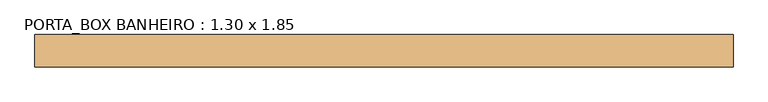
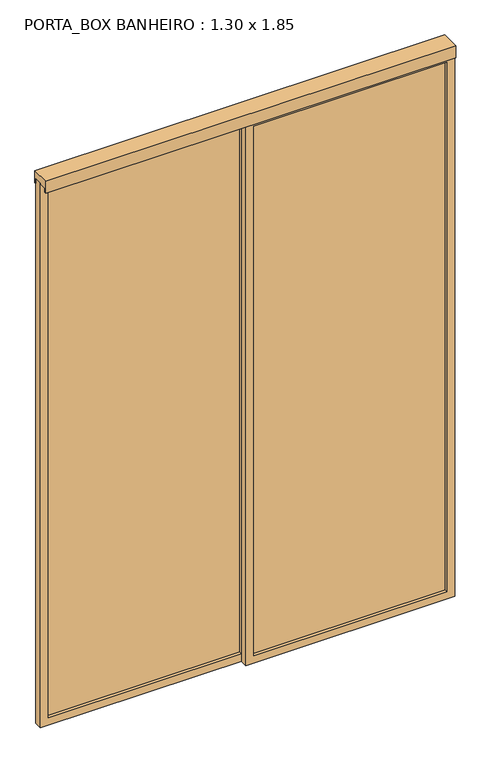
"""IFC4 building model written with IfcOpenShell, lengths in millimetres: door geometry, PORTA_BOX BANHEIRO : 1.30 x 1.85."""

import ifcopenshell
import ifcopenshell.guid

model = None  # the IFC model being written
_history = None  # IfcOwnerHistory: only IFC2X3 demands one
_inside = {}  # id of a spatial element -> (the spatial element, [elements in it])
_under = {}  # id of a project, library or spatial element -> (it, [spatial elements below it])
_declared = {}  # id of a project -> (the project, [libraries it declares])
_typed = {}  # id of a type object -> (the type object, [elements of that type])
_made_of = {}  # id of a material, layer set ... -> (it, [elements and type objects made of it])


def new_model(schema):
    """Start an empty IFC model of exactly this schema.

    Asked for "IFC4X3", IfcOpenShell would pick the latest addendum, in which some entities
    have other attributes; the version numbers below select the first issue.
    IFC2X3 requires an IfcOwnerHistory on every rooted entity: one is made here for all.
    """
    global model, _history
    if schema == "IFC4X3":
        model = ifcopenshell.file(schema_version=(4, 3, 0, 0))
    else:
        model = ifcopenshell.file(schema=schema)
    _inside.clear()
    _under.clear()
    _declared.clear()
    _typed.clear()
    _made_of.clear()
    _history = None
    if model.schema == "IFC2X3":
        org = make("IfcOrganization", Name="unknown")
        user = make(
            "IfcPersonAndOrganization",
            ThePerson=make("IfcPerson", FamilyName="unknown"),
            TheOrganization=org,
        )
        app = make(
            "IfcApplication",
            ApplicationDeveloper=org,
            Version="unknown",
            ApplicationFullName="unknown",
            ApplicationIdentifier="unknown",
        )
        _history = make(
            "IfcOwnerHistory",
            OwningUser=user,
            OwningApplication=app,
            ChangeAction="ADDED",
            CreationDate=0,
        )
    return model


def make(cls, **values):
    """One entity of the class cls with the attributes given. An attribute that is None is left unset."""
    return model.create_entity(
        cls, **{name: value for name, value in values.items() if value is not None}
    )


def rooted(cls, **values):
    """An entity with a GlobalId (a new one), such as an element, a storey or a relation."""
    return make(cls, GlobalId=ifcopenshell.guid.new(), OwnerHistory=_history, **values)


def si_unit(unit_type, name, prefix=None):
    """IfcSIUnit, for example si_unit("LENGTHUNIT", "METRE", prefix="MILLI")."""
    return make("IfcSIUnit", UnitType=unit_type, Prefix=prefix, Name=name)


def assignment(units):
    """IfcUnitAssignment: the units of a project."""
    return None if units is None else make("IfcUnitAssignment", Units=units)


def point(xyz):
    """IfcCartesianPoint."""
    return None if xyz is None else make("IfcCartesianPoint", Coordinates=xyz)


def direction(xyz):
    """IfcDirection."""
    return None if xyz is None else make("IfcDirection", DirectionRatios=xyz)


def frame(location, z_axis=None, x_axis=None):
    """IfcAxis2Placement3D, a coordinate frame: its origin and axes. An axis left out is left unset."""
    return make(
        "IfcAxis2Placement3D",
        Location=point(location),
        Axis=direction(z_axis),
        RefDirection=direction(x_axis),
    )


def origin():
    """The frame at (0, 0, 0) with its axes left unset."""
    return frame((0.0, 0.0, 0.0))


def place(relative_to, where):
    """IfcLocalPlacement: puts the frame where relative to a parent placement (None: the world)."""
    return make(
        "IfcLocalPlacement", PlacementRelTo=relative_to, RelativePlacement=where
    )


def context(
    kind, dimensions, precision=None, world=None, true_north=None, identifier=None
):
    """IfcGeometricRepresentationContext, for example the 3D "Model" context."""
    return make(
        "IfcGeometricRepresentationContext",
        ContextIdentifier=identifier,
        ContextType=kind,
        CoordinateSpaceDimension=dimensions,
        Precision=precision,
        WorldCoordinateSystem=world,
        TrueNorth=true_north,
    )


def project(units=None, contexts=None):
    """IfcProject with its units and contexts."""
    return rooted(
        "IfcProject",
        Name="project",
        RepresentationContexts=contexts,
        UnitsInContext=assignment(units),
    )


def spatial(cls, under=None, at=None, **own):
    """A site, building, storey or space (cls), placed at a placement, below another one or the project."""
    s = rooted(cls, ObjectPlacement=at, **own)
    if under is not None:
        _under.setdefault(under.id(), (under, []))[1].append(s)
    return s


def polyline(points):
    """IfcPolyline through the points."""
    return make("IfcPolyline", Points=[point(p) for p in points])


def outline(outer, holes=None, kind="AREA"):
    """IfcArbitraryClosedProfileDef: a profile drawn as a closed curve; with holes, ...WithVoids."""
    if holes is None:
        return make("IfcArbitraryClosedProfileDef", ProfileType=kind, OuterCurve=outer)
    return make(
        "IfcArbitraryProfileDefWithVoids",
        ProfileType=kind,
        OuterCurve=outer,
        InnerCurves=holes,
    )


def extrude(swept, where, along, depth):
    """IfcExtrudedAreaSolid: the profile swept, set in the frame where, extruded along a direction by depth."""
    return make(
        "IfcExtrudedAreaSolid",
        SweptArea=swept,
        Position=where,
        ExtrudedDirection=direction(along),
        Depth=depth,
    )


def faces_of(points, faces, orient=None, outer=None):
    """IfcFace entities. A face is a list of loops; a loop is a list of indices into points, from 0.

    orient and outer hold one flag for each loop. By default every Orientation is true, the
    first loop of a face is its IfcFaceOuterBound and the others are IfcFaceBound.
    """
    made = []
    for i, loops in enumerate(faces):
        bounds = []
        for j, loop in enumerate(loops):
            is_outer = j == 0 if outer is None else outer[i][j]
            bounds.append(
                make(
                    "IfcFaceOuterBound" if is_outer else "IfcFaceBound",
                    Bound=make("IfcPolyLoop", Polygon=[points[k] for k in loop]),
                    Orientation=True if orient is None else orient[i][j],
                )
            )
        made.append(make("IfcFace", Bounds=bounds))
    return made


def faceted_brep(points, faces, orient=None, outer=None, voids=None):
    """IfcFacetedBrep: a solid bounded by flat faces; with voids (closed shells), ...WithVoids."""
    shared = [point(p) for p in points]
    hull = make("IfcClosedShell", CfsFaces=faces_of(shared, faces, orient, outer))
    if voids is None:
        return make("IfcFacetedBrep", Outer=hull)
    return make(
        "IfcFacetedBrepWithVoids",
        Outer=hull,
        Voids=[
            make(cls, CfsFaces=faces_of(shared, fs, o, b)) for cls, fs, o, b in voids
        ],
    )


def shape(context_of_items, identifier, shape_type, items):
    """IfcShapeRepresentation: the items that make up one representation, for example the "Body"."""
    return make(
        "IfcShapeRepresentation",
        ContextOfItems=context_of_items,
        RepresentationIdentifier=identifier,
        RepresentationType=shape_type,
        Items=items,
    )


def source(mapping_origin, context_of_items, identifier, shape_type, items):
    """IfcRepresentationMap: a shape defined once, which mapped items show again and again."""
    return make(
        "IfcRepresentationMap",
        MappingOrigin=mapping_origin,
        MappedRepresentation=shape(context_of_items, identifier, shape_type, items),
    )


def transform(
    local_origin,
    x_axis=None,
    y_axis=None,
    z_axis=None,
    scale=None,
    scale2=None,
    scale3=None,
    uniform=True,
):
    """IfcCartesianTransformationOperator3D, or its non-uniform kind. x_axis, y_axis, z_axis: its Axis1, 2, 3."""
    if uniform:
        return make(
            "IfcCartesianTransformationOperator3D",
            Axis1=direction(x_axis),
            Axis2=direction(y_axis),
            LocalOrigin=point(local_origin),
            Scale=scale,
            Axis3=direction(z_axis),
        )
    return make(
        "IfcCartesianTransformationOperator3DnonUniform",
        Axis1=direction(x_axis),
        Axis2=direction(y_axis),
        LocalOrigin=point(local_origin),
        Scale=scale,
        Axis3=direction(z_axis),
        Scale2=scale2,
        Scale3=scale3,
    )


def mapped(mapping_source, mapping_target):
    """IfcMappedItem: shows the shape of a source again, moved by a transform."""
    return make(
        "IfcMappedItem", MappingSource=mapping_source, MappingTarget=mapping_target
    )


def made_of(thing, what):
    """Note that an element or type object is made of a material, layer set ...; save() writes the relation."""
    if what is not None:
        _made_of.setdefault(what.id(), (what, []))[1].append(thing)
    return thing


def element(
    cls,
    number,
    at=None,
    inside=None,
    cuts=None,
    type_object=None,
    material=None,
    context=None,
    identifier="Body",
    shape_type=None,
    held_by="IfcProductDefinitionShape",
    body=None,
    shapes=None,
    **own,
):
    """One element of the class cls, such as IfcWall. Its Tag is "e" and its number.

    at: its placement. inside: the storey or other place that contains it. cuts: it is an
    opening in that element (IfcRelVoidsElement). A single representation is given by context,
    identifier, shape_type and body (its items); several are given by shapes. held_by: the class
    of the entity that holds the representations. save() writes the other relations.
    """
    e = rooted(cls, Tag="e%d" % number, ObjectPlacement=at, **own)
    if body is not None:
        shapes = [shape(context, identifier, shape_type, body)]
    if shapes is not None:
        e.Representation = make(held_by, Representations=shapes)
    if inside is not None:
        _inside.setdefault(inside.id(), (inside, []))[1].append(e)
    if cuts is not None:
        rooted(
            "IfcRelVoidsElement", RelatingBuildingElement=cuts, RelatedOpeningElement=e
        )
    if type_object is not None:
        _typed.setdefault(type_object.id(), (type_object, []))[1].append(e)
    return made_of(e, material)


def aggregate(whole, parts):
    """IfcRelAggregates: a whole, such as a stair, and the parts it consists of."""
    return rooted("IfcRelAggregates", RelatingObject=whole, RelatedObjects=parts)


def save(model, path):
    """Write the relations noted so far, then the file.

    IfcRelAggregates (storeys below a building ...), IfcRelContainedInSpatialStructure (elements
    in a storey), IfcRelDefinesByType, IfcRelAssociatesMaterial and IfcRelDeclares: one each for
    every whole, place, type object, material and project.
    """
    for whole, parts in _under.values():
        aggregate(whole, parts)
    for where, things in _inside.values():
        rooted(
            "IfcRelContainedInSpatialStructure",
            RelatedElements=things,
            RelatingStructure=where,
        )
    for kind, things in _typed.values():
        rooted("IfcRelDefinesByType", RelatedObjects=things, RelatingType=kind)
    for what, things in _made_of.values():
        rooted("IfcRelAssociatesMaterial", RelatedObjects=things, RelatingMaterial=what)
    for by, libraries in _declared.values():
        rooted("IfcRelDeclares", RelatingContext=by, RelatedDefinitions=libraries)
    model.write(path)


def porta_box_banheiro_1_30_x_1_85_9eacd337(model_context):
    return source(origin(), model_context, "Body", "SolidModel", [
        extrude(outline(polyline([(652.5, -15.0), (10.0, -15.0), (10.0, -10.0), (652.5, -10.0), (652.5, -15.0)])), frame((0.0, 0.0, 10.0), z_axis=(0.0, 0.0, 1.0), x_axis=(1.0, 0.0, 0.0)), (0.0, 0.0, 1.0), 1805.0),
        faceted_brep([(637.5, -15.0, 1800.0), (637.5, -15.0, 25.0), (637.5, -25.0, 25.0), (637.5, -25.0, 1800.0), (662.5, -25.0, 1825.0), (0.0, -25.0, 1825.0), (0.0, -25.0, 0.0), (662.5, -25.0, 0.0), (25.0, -25.0, 1800.0), (25.0, -25.0, 25.0), (25.0, -15.0, 25.0), (10.0, -15.0, 1815.0), (652.5, -15.0, 1815.0), (652.5, -15.0, 10.0), (10.0, -15.0, 10.0), (25.0, -15.0, 1800.0), (662.5, 0.0, 0.0), (662.5, 0.0, 1825.0), (0.0, 0.0, 1825.0), (0.0, 0.0, 0.0), (637.5, 0.0, 1800.0), (25.0, 0.0, 1800.0), (25.0, 0.0, 25.0), (637.5, 0.0, 25.0), (637.5, -10.0, 25.0), (637.5, -10.0, 1800.0), (25.0, -10.0, 25.0), (25.0, -10.0, 1800.0), (652.5, -10.0, 1815.0), (652.5, -10.0, 10.0), (10.0, -10.0, 10.0), (10.0, -10.0, 1815.0)], [[[0, 1, 2, 3]], [[4, 5, 6, 7], [8, 3, 2, 9]], [[1, 10, 9, 2]], [[11, 12, 13, 14], [0, 15, 10, 1]], [[4, 7, 16, 17]], [[18, 17, 16, 19], [20, 21, 22, 23]], [[7, 6, 19, 16]], [[10, 15, 8, 9]], [[6, 5, 18, 19]], [[20, 23, 24, 25]], [[23, 22, 26, 24]], [[22, 21, 27, 26]], [[28, 29, 13, 12]], [[29, 30, 14, 13]], [[28, 31, 30, 29], [27, 25, 24, 26]], [[30, 31, 11, 14]], [[15, 0, 3, 8]], [[5, 4, 17, 18]], [[31, 28, 12, 11]], [[21, 20, 25, 27]]]),
        extrude(outline(polyline([(1290.0, -40.0), (647.5, -40.0), (647.5, -35.0), (1290.0, -35.0), (1290.0, -40.0)])), frame((0.0, 0.0, 10.0), z_axis=(0.0, 0.0, 1.0), x_axis=(1.0, 0.0, 0.0)), (0.0, 0.0, 1.0), 1805.0),
        faceted_brep([(1275.0, -40.0, 1800.0), (1275.0, -40.0, 25.0), (1275.0, -50.0, 25.0), (1275.0, -50.0, 1800.0), (1300.0, -50.0, 1825.0), (637.5, -50.0, 1825.0), (637.5, -50.0, 0.0), (1300.0, -50.0, 0.0), (662.5, -50.0, 1800.0), (662.5, -50.0, 25.0), (662.5, -40.0, 25.0), (647.5, -40.0, 1815.0), (1290.0, -40.0, 1815.0), (1290.0, -40.0, 10.0), (647.5, -40.0, 10.0), (662.5, -40.0, 1800.0), (1300.0, -25.0, 0.0), (1300.0, -25.0, 1825.0), (637.5, -25.0, 1825.0), (637.5, -25.0, 0.0), (1275.0, -25.0, 1800.0), (662.5, -25.0, 1800.0), (662.5, -25.0, 25.0), (1275.0, -25.0, 25.0), (1275.0, -35.0, 25.0), (1275.0, -35.0, 1800.0), (662.5, -35.0, 25.0), (662.5, -35.0, 1800.0), (1290.0, -35.0, 1815.0), (1290.0, -35.0, 10.0), (647.5, -35.0, 10.0), (647.5, -35.0, 1815.0)], [[[0, 1, 2, 3]], [[4, 5, 6, 7], [8, 3, 2, 9]], [[1, 10, 9, 2]], [[11, 12, 13, 14], [0, 15, 10, 1]], [[4, 7, 16, 17]], [[18, 17, 16, 19], [20, 21, 22, 23]], [[7, 6, 19, 16]], [[10, 15, 8, 9]], [[6, 5, 18, 19]], [[20, 23, 24, 25]], [[23, 22, 26, 24]], [[22, 21, 27, 26]], [[28, 29, 13, 12]], [[29, 30, 14, 13]], [[28, 31, 30, 29], [27, 25, 24, 26]], [[30, 31, 11, 14]], [[15, 0, 3, 8]], [[5, 4, 17, 18]], [[31, 28, 12, 11]], [[21, 20, 25, 27]]]),
        extrude(outline(polyline([(5.0, 1810.0), (0.0, 1810.0), (0.0, 1825.0), (-50.0, 1825.0), (-50.0, 1810.0), (-55.0, 1810.0), (-55.0, 1850.0), (5.0, 1850.0), (5.0, 1810.0)])), frame((0.0, 0.0, 0.0), z_axis=(1.0, 0.0, 0.0), x_axis=(0.0, 1.0, 0.0)), (0.0, 0.0, 1.0), 1300.0),
    ])


if __name__ == "__main__":
    model = new_model("IFC4")
    model_context = context("Model", 3, world=origin())
    ifc_project = project(units=[si_unit("LENGTHUNIT", "METRE", prefix="MILLI")], contexts=[model_context])
    site = spatial("IfcSite", under=ifc_project)
    building = spatial("IfcBuilding", under=site)
    placement = place(None, origin())
    porta_box_banheiro_1_30_x_1_85_shape = porta_box_banheiro_1_30_x_1_85_9eacd337(model_context)
    element("IfcDoor", 1, ObjectType="PORTA_BOX BANHEIRO : 1.30 x 1.85", at=placement, inside=building, context=model_context, shape_type="MappedRepresentation", body=[
        mapped(porta_box_banheiro_1_30_x_1_85_shape, transform((0.0, 0.0, 0.0), x_axis=(1.0, 0.0, 0.0), y_axis=(0.0, 1.0, 0.0), z_axis=(0.0, 0.0, 1.0))),
    ])
    save(model, "model.ifc")

# Revit data of these elements
# Type "PORTA_BOX BANHEIRO : 1.30 x 1.85"
#   Type Mark = "BOX"
#   Width = 1.30 m
#   Material montante = .ALUMÍNIO
#   Materia vidro = .VIDRO
# Element 1 (IfcDoor, "PORTA_BOX BANHEIRO : 1.30 x 1.85")
#   Materials on its faces: ".ALUMÍNIO", ".VIDRO"
# Materials
#   ".ALUMÍNIO": class "CC_METAIS", colour RGB 244 244 244, transparency 0, Description = "Material alumínio", Cost = 0
#   ".VIDRO": class "Genérico", colour RGB 198 236 255, transparency 0.95, Cost = 0
